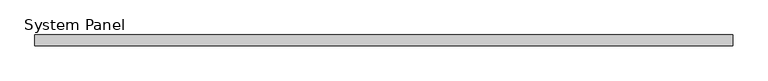
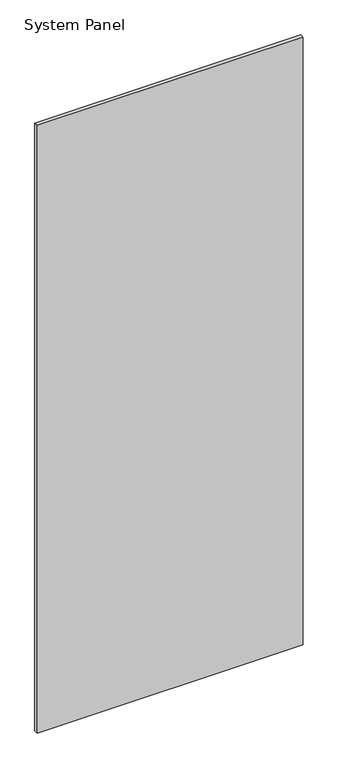
"""IFC4 building model written with IfcOpenShell, lengths in millimetres: plate geometry, System Panel : WWm-Glass-20mm-10mmOffset."""

from ifc_helpers import new_model, si_unit, origin, origin_with_axes, place, context, project, spatial, polyline, outline, extrude, source, transform, mapped, element, save


def system_panel_1e2ea1b5(model_context):
    return source(origin(), model_context, "Body", "SweptSolid", [
        extrude(outline(polyline([(652.5, 0.0), (-652.5, 0.0), (-652.5, 20.0), (652.5, 20.0), (652.5, 0.0)])), origin_with_axes(), (0.0, 0.0, 1.0), 3150.0),
    ])


if __name__ == "__main__":
    model = new_model("IFC4")
    model_context = context("Model", 3, world=origin())
    ifc_project = project(units=[si_unit("LENGTHUNIT", "METRE", prefix="MILLI")], contexts=[model_context])
    site = spatial("IfcSite", under=ifc_project)
    building = spatial("IfcBuilding", under=site)
    placement = place(None, origin())
    system_panel_shape = system_panel_1e2ea1b5(model_context)
    element("IfcPlate", 1, ObjectType="System Panel : WWm-Glass-20mm-10mmOffset", at=placement, inside=building, context=model_context, shape_type="MappedRepresentation", body=[
        mapped(system_panel_shape, transform((0.0, 0.0, 0.0), x_axis=(1.0, 0.0, 0.0), y_axis=(0.0, 1.0, 0.0), z_axis=(0.0, 0.0, 1.0))),
    ])
    save(model, "model.ifc")

# Revit data of these elements
# Type "System Panel : WWm-Glass-20mm-10mmOffset"
#   Finish = ""
# Element 1 (IfcPlate, "System Panel : WWm-Glass-20mm-10mmOffset")
#   Materials on its faces: "WW-EC-GL-Storefront"
# Materials
#   "WW-EC-GL-Storefront": class "Glass", colour RGB 236 240 239, transparency 0.85, Description = "Storefront Glass", Cost = 0
